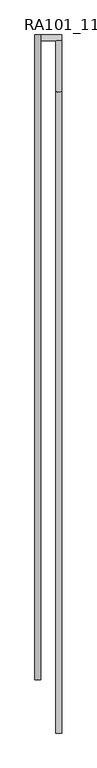
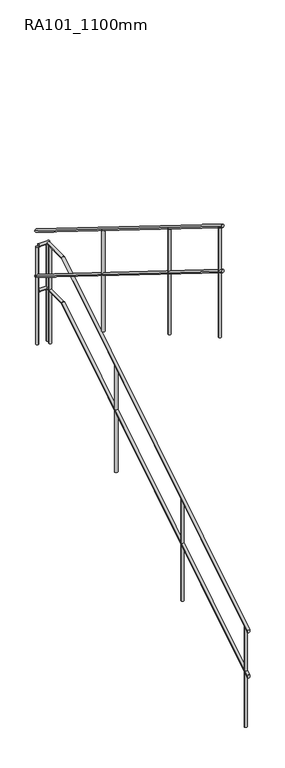
"""IFC4 building model written with IfcOpenShell, lengths in millimetres: railing geometry, RA101_1100mm."""

import ifcopenshell
import ifcopenshell.guid

model = None  # the IFC model being written
_history = None  # IfcOwnerHistory: only IFC2X3 demands one
_inside = {}  # id of a spatial element -> (the spatial element, [elements in it])
_under = {}  # id of a project, library or spatial element -> (it, [spatial elements below it])
_declared = {}  # id of a project -> (the project, [libraries it declares])
_typed = {}  # id of a type object -> (the type object, [elements of that type])
_made_of = {}  # id of a material, layer set ... -> (it, [elements and type objects made of it])


def new_model(schema):
    """Start an empty IFC model of exactly this schema.

    Asked for "IFC4X3", IfcOpenShell would pick the latest addendum, in which some entities
    have other attributes; the version numbers below select the first issue.
    IFC2X3 requires an IfcOwnerHistory on every rooted entity: one is made here for all.
    """
    global model, _history
    if schema == "IFC4X3":
        model = ifcopenshell.file(schema_version=(4, 3, 0, 0))
    else:
        model = ifcopenshell.file(schema=schema)
    _inside.clear()
    _under.clear()
    _declared.clear()
    _typed.clear()
    _made_of.clear()
    _history = None
    if model.schema == "IFC2X3":
        org = make("IfcOrganization", Name="unknown")
        user = make(
            "IfcPersonAndOrganization",
            ThePerson=make("IfcPerson", FamilyName="unknown"),
            TheOrganization=org,
        )
        app = make(
            "IfcApplication",
            ApplicationDeveloper=org,
            Version="unknown",
            ApplicationFullName="unknown",
            ApplicationIdentifier="unknown",
        )
        _history = make(
            "IfcOwnerHistory",
            OwningUser=user,
            OwningApplication=app,
            ChangeAction="ADDED",
            CreationDate=0,
        )
    return model


def make(cls, **values):
    """One entity of the class cls with the attributes given. An attribute that is None is left unset."""
    return model.create_entity(
        cls, **{name: value for name, value in values.items() if value is not None}
    )


def rooted(cls, **values):
    """An entity with a GlobalId (a new one), such as an element, a storey or a relation."""
    return make(cls, GlobalId=ifcopenshell.guid.new(), OwnerHistory=_history, **values)


def si_unit(unit_type, name, prefix=None):
    """IfcSIUnit, for example si_unit("LENGTHUNIT", "METRE", prefix="MILLI")."""
    return make("IfcSIUnit", UnitType=unit_type, Prefix=prefix, Name=name)


def assignment(units):
    """IfcUnitAssignment: the units of a project."""
    return None if units is None else make("IfcUnitAssignment", Units=units)


def point(xyz):
    """IfcCartesianPoint."""
    return None if xyz is None else make("IfcCartesianPoint", Coordinates=xyz)


def direction(xyz):
    """IfcDirection."""
    return None if xyz is None else make("IfcDirection", DirectionRatios=xyz)


def frame(location, z_axis=None, x_axis=None):
    """IfcAxis2Placement3D, a coordinate frame: its origin and axes. An axis left out is left unset."""
    return make(
        "IfcAxis2Placement3D",
        Location=point(location),
        Axis=direction(z_axis),
        RefDirection=direction(x_axis),
    )


def frame_2d(location, x_axis=None):
    """IfcAxis2Placement2D, a coordinate frame in the plane: its origin and x axis."""
    return make(
        "IfcAxis2Placement2D", Location=point(location), RefDirection=direction(x_axis)
    )


def origin():
    """The frame at (0, 0, 0) with its axes left unset."""
    return frame((0.0, 0.0, 0.0))


def place(relative_to, where):
    """IfcLocalPlacement: puts the frame where relative to a parent placement (None: the world)."""
    return make(
        "IfcLocalPlacement", PlacementRelTo=relative_to, RelativePlacement=where
    )


def context(
    kind, dimensions, precision=None, world=None, true_north=None, identifier=None
):
    """IfcGeometricRepresentationContext, for example the 3D "Model" context."""
    return make(
        "IfcGeometricRepresentationContext",
        ContextIdentifier=identifier,
        ContextType=kind,
        CoordinateSpaceDimension=dimensions,
        Precision=precision,
        WorldCoordinateSystem=world,
        TrueNorth=true_north,
    )


def project(units=None, contexts=None):
    """IfcProject with its units and contexts."""
    return rooted(
        "IfcProject",
        Name="project",
        RepresentationContexts=contexts,
        UnitsInContext=assignment(units),
    )


def spatial(cls, under=None, at=None, **own):
    """A site, building, storey or space (cls), placed at a placement, below another one or the project."""
    s = rooted(cls, ObjectPlacement=at, **own)
    if under is not None:
        _under.setdefault(under.id(), (under, []))[1].append(s)
    return s


def circle_curve(where, radius):
    """IfcCircle in the frame where."""
    return make("IfcCircle", Position=where, Radius=radius)


def ellipse_curve(where, semi_axis1, semi_axis2):
    """IfcEllipse in the frame where."""
    return make(
        "IfcEllipse", Position=where, SemiAxis1=semi_axis1, SemiAxis2=semi_axis2
    )


def trimmed(basis, trim1, trim2, sense, master):
    """IfcTrimmedCurve: the piece of a basis curve between two trims."""
    return make(
        "IfcTrimmedCurve",
        BasisCurve=basis,
        Trim1=trim1,
        Trim2=trim2,
        SenseAgreement=sense,
        MasterRepresentation=master,
    )


def segment(curve, same_sense, transition):
    """IfcCompositeCurveSegment."""
    return make(
        "IfcCompositeCurveSegment",
        Transition=transition,
        SameSense=same_sense,
        ParentCurve=curve,
    )


def composite_curve(segments, self_intersect=None):
    """IfcCompositeCurve: segments joined end to end."""
    return make("IfcCompositeCurve", Segments=segments, SelfIntersect=self_intersect)


def outline(outer, holes=None, kind="AREA"):
    """IfcArbitraryClosedProfileDef: a profile drawn as a closed curve; with holes, ...WithVoids."""
    if holes is None:
        return make("IfcArbitraryClosedProfileDef", ProfileType=kind, OuterCurve=outer)
    return make(
        "IfcArbitraryProfileDefWithVoids",
        ProfileType=kind,
        OuterCurve=outer,
        InnerCurves=holes,
    )


def extrude(swept, where, along, depth):
    """IfcExtrudedAreaSolid: the profile swept, set in the frame where, extruded along a direction by depth."""
    return make(
        "IfcExtrudedAreaSolid",
        SweptArea=swept,
        Position=where,
        ExtrudedDirection=direction(along),
        Depth=depth,
    )


def shape(context_of_items, identifier, shape_type, items):
    """IfcShapeRepresentation: the items that make up one representation, for example the "Body"."""
    return make(
        "IfcShapeRepresentation",
        ContextOfItems=context_of_items,
        RepresentationIdentifier=identifier,
        RepresentationType=shape_type,
        Items=items,
    )


def source(mapping_origin, context_of_items, identifier, shape_type, items):
    """IfcRepresentationMap: a shape defined once, which mapped items show again and again."""
    return make(
        "IfcRepresentationMap",
        MappingOrigin=mapping_origin,
        MappedRepresentation=shape(context_of_items, identifier, shape_type, items),
    )


def transform(
    local_origin,
    x_axis=None,
    y_axis=None,
    z_axis=None,
    scale=None,
    scale2=None,
    scale3=None,
    uniform=True,
):
    """IfcCartesianTransformationOperator3D, or its non-uniform kind. x_axis, y_axis, z_axis: its Axis1, 2, 3."""
    if uniform:
        return make(
            "IfcCartesianTransformationOperator3D",
            Axis1=direction(x_axis),
            Axis2=direction(y_axis),
            LocalOrigin=point(local_origin),
            Scale=scale,
            Axis3=direction(z_axis),
        )
    return make(
        "IfcCartesianTransformationOperator3DnonUniform",
        Axis1=direction(x_axis),
        Axis2=direction(y_axis),
        LocalOrigin=point(local_origin),
        Scale=scale,
        Axis3=direction(z_axis),
        Scale2=scale2,
        Scale3=scale3,
    )


def mapped(mapping_source, mapping_target):
    """IfcMappedItem: shows the shape of a source again, moved by a transform."""
    return make(
        "IfcMappedItem", MappingSource=mapping_source, MappingTarget=mapping_target
    )


def made_of(thing, what):
    """Note that an element or type object is made of a material, layer set ...; save() writes the relation."""
    if what is not None:
        _made_of.setdefault(what.id(), (what, []))[1].append(thing)
    return thing


def element(
    cls,
    number,
    at=None,
    inside=None,
    cuts=None,
    type_object=None,
    material=None,
    context=None,
    identifier="Body",
    shape_type=None,
    held_by="IfcProductDefinitionShape",
    body=None,
    shapes=None,
    **own,
):
    """One element of the class cls, such as IfcWall. Its Tag is "e" and its number.

    at: its placement. inside: the storey or other place that contains it. cuts: it is an
    opening in that element (IfcRelVoidsElement). A single representation is given by context,
    identifier, shape_type and body (its items); several are given by shapes. held_by: the class
    of the entity that holds the representations. save() writes the other relations.
    """
    e = rooted(cls, Tag="e%d" % number, ObjectPlacement=at, **own)
    if body is not None:
        shapes = [shape(context, identifier, shape_type, body)]
    if shapes is not None:
        e.Representation = make(held_by, Representations=shapes)
    if inside is not None:
        _inside.setdefault(inside.id(), (inside, []))[1].append(e)
    if cuts is not None:
        rooted(
            "IfcRelVoidsElement", RelatingBuildingElement=cuts, RelatedOpeningElement=e
        )
    if type_object is not None:
        _typed.setdefault(type_object.id(), (type_object, []))[1].append(e)
    return made_of(e, material)


def aggregate(whole, parts):
    """IfcRelAggregates: a whole, such as a stair, and the parts it consists of."""
    return rooted("IfcRelAggregates", RelatingObject=whole, RelatedObjects=parts)


def save(model, path):
    """Write the relations noted so far, then the file.

    IfcRelAggregates (storeys below a building ...), IfcRelContainedInSpatialStructure (elements
    in a storey), IfcRelDefinesByType, IfcRelAssociatesMaterial and IfcRelDeclares: one each for
    every whole, place, type object, material and project.
    """
    for whole, parts in _under.values():
        aggregate(whole, parts)
    for where, things in _inside.values():
        rooted(
            "IfcRelContainedInSpatialStructure",
            RelatedElements=things,
            RelatingStructure=where,
        )
    for kind, things in _typed.values():
        rooted("IfcRelDefinesByType", RelatedObjects=things, RelatingType=kind)
    for what, things in _made_of.values():
        rooted("IfcRelAssociatesMaterial", RelatedObjects=things, RelatingMaterial=what)
    for by, libraries in _declared.values():
        rooted("IfcRelDeclares", RelatingContext=by, RelatedDefinitions=libraries)
    model.write(path)


def plane_surface(at):
    """IfcPlane: the flat surface through the origin of the frame at, square to its z axis."""
    return make("IfcPlane", Position=at)


def cylinder_surface(at, radius):
    """IfcCylindricalSurface: all points at the distance radius from the z axis of the frame at."""
    return make("IfcCylindricalSurface", Position=at, Radius=radius)


def advanced_brep(points, edges, surfaces, faces):
    """IfcAdvancedBrep: a solid bounded by faces that lie on surfaces and meet in shared edges.

    An edge is (start, end): straight between two places in points (the first is 0);
    or (start, end, curve); or (start, end, curve, False) where it runs against its curve.
    A face is (place in surfaces, loops), or (place, loops, False) where it looks against
    its surface's normal. A loop lists edges by number (the first is 1), with a minus sign
    where the edge is run from its end to its start. The first loop is the outer one.
    """
    corners = [point(p) for p in points]
    vertices = [make("IfcVertexPoint", VertexGeometry=c) for c in corners]
    made = []
    for start, end, *more in edges:
        made.append(
            make(
                "IfcEdgeCurve",
                EdgeStart=vertices[start],
                EdgeEnd=vertices[end],
                EdgeGeometry=more[0] if more else make("IfcPolyline", Points=[corners[start], corners[end]]),
                SameSense=more[1] if len(more) > 1 else True,
            )
        )
    hull = []
    for where, loops, *sense in faces:
        bounds = []
        for j, loop in enumerate(loops):
            ring = [make("IfcOrientedEdge", EdgeElement=made[abs(k) - 1], Orientation=k > 0) for k in loop]
            bounds.append(
                make(
                    "IfcFaceOuterBound" if j == 0 else "IfcFaceBound",
                    Bound=make("IfcEdgeLoop", EdgeList=ring),
                    Orientation=True,
                )
            )
        hull.append(make("IfcAdvancedFace", Bounds=bounds, FaceSurface=surfaces[where], SameSense=sense[0] if sense else True))
    return make("IfcAdvancedBrep", Outer=make("IfcClosedShell", CfsFaces=hull))


def ra101_1100mm_1ac2519f(model_context):
    return source(origin(), model_context, "Body", "SolidModel", [
        advanced_brep(
        [(11545.1052251, 14699.5208589, 456.3396197), (11515.1052251, 14699.5208589, 456.3396197), (11545.1052251, 18329.5208589, 2547.0), (11515.1052251, 18329.5208589, 2547.0), (11545.1052251, 18063.8019306, 2547.0), (11515.1052251, 18063.8019306, 2547.0)],
        [
            (0, 1, ellipse_curve(frame((11530.1052251, 14699.5208589, 456.3396197), z_axis=(0.0, -1.0, 0.0), x_axis=(0.0, 0.0, -1.0)), 17.6603803, 15.0)),
            (1, 0, ellipse_curve(frame((11530.1052251, 14699.5208589, 456.3396197), z_axis=(0.0, -1.0, 0.0), x_axis=(0.0, 0.0, -1.0)), 17.6603803, 15.0)),
            (2, 3, circle_curve(frame((11530.1052251, 18329.5208589, 2547.0), z_axis=(0.0, 1.0, 0.0), x_axis=(-1.0, 0.0, 0.0)), 15.0)),
            (3, 2, circle_curve(frame((11530.1052251, 18329.5208589, 2547.0), z_axis=(0.0, 1.0, 0.0), x_axis=(-1.0, 0.0, 0.0)), 15.0)),
            (0, 4),
            (4, 5, ellipse_curve(frame((11530.1052251, 18063.8019306, 2547.0), z_axis=(0.0, -0.9616025257983003, -0.2744459552959912), x_axis=(0.0, 0.2744459552959914, -0.9616025257983002)), 15.5989607, 15.0)),
            (5, 1),
            (5, 4, ellipse_curve(frame((11530.1052251, 18063.8019306, 2547.0), z_axis=(0.0, -0.9616025257983003, -0.2744459552959912), x_axis=(0.0, 0.2744459552959914, -0.9616025257983002)), 15.5989607, 15.0)),
            (4, 2),
            (3, 5),
        ],
        [
            plane_surface(frame((11530.1052251, 14699.5208589, 474.0), z_axis=(0.0, -1.0, 0.0), x_axis=(0.0, 0.0, 1.0))),
            plane_surface(frame((11530.1052251, 18329.5208589, 2562.0), z_axis=(0.0, 1.0, 0.0), x_axis=(0.0, 0.0, 1.0))),
            cylinder_surface(frame((11530.1052251, 14707.4380966, 461.2596175), z_axis=(0.0, -0.8493588352433417, -0.5278158476155052), x_axis=(-1.0, 0.0, 0.0)), 15.0),
            cylinder_surface(frame((11530.1052251, 18059.5208589, 2547.0), z_axis=(0.0, -1.0, 0.0), x_axis=(-1.0, 0.0, 0.0)), 15.0),
        ],
        [
            (0, [[1, 2]]),
            (1, [[3, 4]]),
            (2, [[-1, 5, 6, 7]]),
            (2, [[-2, -7, 8, -5]]),
            (3, [[-6, 9, -4, 10]]),
            (3, [[-8, -10, -3, -9]]),
        ],
    ),
        advanced_brep(
        [(11545.1052251, 18359.5208589, 2547.0), (11545.1052251, 18329.5208589, 2547.0), (11435.1052251, 18359.5208589, 2547.0), (11435.1052251, 18329.5208589, 2547.0)],
        [
            (0, 1, circle_curve(frame((11545.1052251, 18344.5208589, 2547.0), z_axis=(1.0, 0.0, 0.0), x_axis=(0.0, -1.0, 0.0)), 15.0)),
            (1, 0, circle_curve(frame((11545.1052251, 18344.5208589, 2547.0), z_axis=(1.0, 0.0, 0.0), x_axis=(0.0, -1.0, 0.0)), 15.0)),
            (2, 3, circle_curve(frame((11435.1052251, 18344.5208589, 2547.0), z_axis=(-1.0, 0.0, 0.0), x_axis=(0.0, -1.0, 0.0)), 15.0)),
            (3, 2, circle_curve(frame((11435.1052251, 18344.5208589, 2547.0), z_axis=(-1.0, 0.0, 0.0), x_axis=(0.0, -1.0, 0.0)), 15.0)),
            (0, 2),
            (3, 1),
        ],
        [
            plane_surface(frame((11545.1052251, 18344.5208589, 2562.0), z_axis=(1.0, 0.0, 0.0), x_axis=(0.0, -1.0, 0.0))),
            plane_surface(frame((11435.1052251, 18344.5208589, 2562.0), z_axis=(-1.0, 0.0, 0.0), x_axis=(0.0, -1.0, 0.0))),
            cylinder_surface(frame((11545.1052251, 18344.5208589, 2547.0), z_axis=(1.0, 0.0, 0.0), x_axis=(0.0, -1.0, 0.0)), 15.0),
        ],
        [
            (0, [[1, 2]]),
            (1, [[3, 4]]),
            (2, [[-1, 5, -4, 6]]),
            (2, [[-2, -6, -3, -5]]),
        ],
    ),
        advanced_brep(
        [(11405.1052251, 18359.5208589, 2705.9110483), (11435.1052251, 18359.5208589, 2705.9110483), (11405.1052251, 14979.5208589, 4806.3396197), (11435.1052251, 14979.5208589, 4806.3396197)],
        [
            (0, 1, ellipse_curve(frame((11420.1052251, 18359.5208589, 2705.9110483), z_axis=(0.0, 1.0, 0.0), x_axis=(0.0, 0.0, -1.0)), 17.6603803, 15.0)),
            (1, 0, ellipse_curve(frame((11420.1052251, 18359.5208589, 2705.9110483), z_axis=(0.0, 1.0, 0.0), x_axis=(0.0, 0.0, -1.0)), 17.6603803, 15.0)),
            (2, 3, ellipse_curve(frame((11420.1052251, 14979.5208589, 4806.3396197), z_axis=(0.0, -1.0, 0.0), x_axis=(0.0, 0.0, -1.0)), 17.6603803, 15.0)),
            (3, 2, ellipse_curve(frame((11420.1052251, 14979.5208589, 4806.3396197), z_axis=(0.0, -1.0, 0.0), x_axis=(0.0, 0.0, -1.0)), 17.6603803, 15.0)),
            (0, 2),
            (3, 1),
        ],
        [
            plane_surface(frame((11420.1052251, 18359.5208589, 2723.5714286), z_axis=(0.0, 1.0, 0.0), x_axis=(0.0, 0.0, -1.0))),
            plane_surface(frame((11420.1052251, 14979.5208589, 4824.0), z_axis=(0.0, -1.0, 0.0), x_axis=(0.0, 0.0, -1.0))),
            cylinder_surface(frame((11420.1052251, 18351.6036212, 2710.831046), z_axis=(0.0, 0.8493588352433417, -0.5278158476155052), x_axis=(1.0, 0.0, 0.0)), 15.0),
        ],
        [
            (0, [[1, 2]]),
            (1, [[3, 4]]),
            (2, [[-1, 5, -4, 6]]),
            (2, [[-2, -6, -3, -5]]),
        ],
    ),
        advanced_brep(
        [(11545.1052251, 14699.5208589, 956.3396197), (11515.1052251, 14699.5208589, 956.3396197), (11545.1052251, 18063.8019306, 3047.0), (11515.1052251, 18063.8019306, 3047.0), (11545.1052251, 18329.5208589, 3047.0), (11515.1052251, 18329.5208589, 3047.0)],
        [
            (0, 1, ellipse_curve(frame((11530.1052251, 14699.5208589, 956.3396197), z_axis=(0.0, -1.0, 0.0), x_axis=(0.0, 0.0, -1.0)), 17.6603803, 15.0)),
            (1, 0, ellipse_curve(frame((11530.1052251, 14699.5208589, 956.3396197), z_axis=(0.0, -1.0, 0.0), x_axis=(0.0, 0.0, -1.0)), 17.6603803, 15.0)),
            (0, 2),
            (2, 3, ellipse_curve(frame((11530.1052251, 18063.8019306, 3047.0), z_axis=(0.0, -0.9616025257983003, -0.2744459552959912), x_axis=(0.0, 0.2744459552959914, -0.9616025257983002)), 15.5989607, 15.0)),
            (3, 1),
            (3, 2, ellipse_curve(frame((11530.1052251, 18063.8019306, 3047.0), z_axis=(0.0, -0.9616025257983003, -0.2744459552959912), x_axis=(0.0, 0.2744459552959914, -0.9616025257983002)), 15.5989607, 15.0)),
            (4, 5, circle_curve(frame((11530.1052251, 18329.5208589, 3047.0), z_axis=(0.0, 1.0, 0.0), x_axis=(-1.0, 0.0, 0.0)), 15.0)),
            (5, 4, circle_curve(frame((11530.1052251, 18329.5208589, 3047.0), z_axis=(0.0, 1.0, 0.0), x_axis=(-1.0, 0.0, 0.0)), 15.0)),
            (2, 4),
            (5, 3),
        ],
        [
            plane_surface(frame((11530.1052251, 14699.5208589, 974.0), z_axis=(0.0, -1.0, 0.0), x_axis=(0.0, 0.0, 1.0))),
            cylinder_surface(frame((11530.1052251, 14707.4380966, 961.2596175), z_axis=(0.0, -0.8493588352433417, -0.5278158476155052), x_axis=(-1.0, 0.0, 0.0)), 15.0),
            plane_surface(frame((11530.1052251, 18329.5208589, 3062.0), z_axis=(0.0, 1.0, 0.0), x_axis=(0.0, 0.0, 1.0))),
            cylinder_surface(frame((11530.1052251, 18059.5208589, 3047.0), z_axis=(0.0, -1.0, 0.0), x_axis=(-1.0, 0.0, 0.0)), 15.0),
        ],
        [
            (0, [[1, 2]]),
            (1, [[-1, 3, 4, 5]]),
            (1, [[-2, -5, 6, -3]]),
            (2, [[7, 8]]),
            (3, [[-4, 9, -8, 10]]),
            (3, [[-6, -10, -7, -9]]),
        ],
    ),
        advanced_brep(
        [(11545.1052251, 18359.5208589, 3047.0), (11545.1052251, 18329.5208589, 3047.0), (11435.1052251, 18359.5208589, 3047.0), (11435.1052251, 18329.5208589, 3047.0)],
        [
            (0, 1, circle_curve(frame((11545.1052251, 18344.5208589, 3047.0), z_axis=(1.0, 0.0, 0.0), x_axis=(0.0, -1.0, 0.0)), 15.0)),
            (1, 0, circle_curve(frame((11545.1052251, 18344.5208589, 3047.0), z_axis=(1.0, 0.0, 0.0), x_axis=(0.0, -1.0, 0.0)), 15.0)),
            (2, 3, circle_curve(frame((11435.1052251, 18344.5208589, 3047.0), z_axis=(-1.0, 0.0, 0.0), x_axis=(0.0, -1.0, 0.0)), 15.0)),
            (3, 2, circle_curve(frame((11435.1052251, 18344.5208589, 3047.0), z_axis=(-1.0, 0.0, 0.0), x_axis=(0.0, -1.0, 0.0)), 15.0)),
            (0, 2),
            (3, 1),
        ],
        [
            plane_surface(frame((11545.1052251, 18344.5208589, 3062.0), z_axis=(1.0, 0.0, 0.0), x_axis=(0.0, -1.0, 0.0))),
            plane_surface(frame((11435.1052251, 18344.5208589, 3062.0), z_axis=(-1.0, 0.0, 0.0), x_axis=(0.0, -1.0, 0.0))),
            cylinder_surface(frame((11545.1052251, 18344.5208589, 3047.0), z_axis=(1.0, 0.0, 0.0), x_axis=(0.0, -1.0, 0.0)), 15.0),
        ],
        [
            (0, [[1, 2]]),
            (1, [[3, 4]]),
            (2, [[-1, 5, -4, 6]]),
            (2, [[-2, -6, -3, -5]]),
        ],
    ),
        advanced_brep(
        [(11405.1052251, 18359.5208589, 3205.9110483), (11435.1052251, 18359.5208589, 3205.9110483), (11405.1052251, 14979.5208589, 5306.3396197), (11435.1052251, 14979.5208589, 5306.3396197)],
        [
            (0, 1, ellipse_curve(frame((11420.1052251, 18359.5208589, 3205.9110483), z_axis=(0.0, 1.0, 0.0), x_axis=(0.0, 0.0, -1.0)), 17.6603803, 15.0)),
            (1, 0, ellipse_curve(frame((11420.1052251, 18359.5208589, 3205.9110483), z_axis=(0.0, 1.0, 0.0), x_axis=(0.0, 0.0, -1.0)), 17.6603803, 15.0)),
            (2, 3, ellipse_curve(frame((11420.1052251, 14979.5208589, 5306.3396197), z_axis=(0.0, -1.0, 0.0), x_axis=(0.0, 0.0, -1.0)), 17.6603803, 15.0)),
            (3, 2, ellipse_curve(frame((11420.1052251, 14979.5208589, 5306.3396197), z_axis=(0.0, -1.0, 0.0), x_axis=(0.0, 0.0, -1.0)), 17.6603803, 15.0)),
            (0, 2),
            (3, 1),
        ],
        [
            plane_surface(frame((11420.1052251, 18359.5208589, 3223.5714286), z_axis=(0.0, 1.0, 0.0), x_axis=(0.0, 0.0, -1.0))),
            plane_surface(frame((11420.1052251, 14979.5208589, 5324.0), z_axis=(0.0, -1.0, 0.0), x_axis=(0.0, 0.0, -1.0))),
            cylinder_surface(frame((11420.1052251, 18351.6036212, 3210.831046), z_axis=(0.0, 0.8493588352433417, -0.5278158476155052), x_axis=(1.0, 0.0, 0.0)), 15.0),
        ],
        [
            (0, [[1, 2]]),
            (1, [[3, 4]]),
            (2, [[-1, 5, -4, 6]]),
            (2, [[-2, -6, -3, -5]]),
        ],
    ),
        extrude(outline(composite_curve([segment(trimmed(circle_curve(frame_2d((11420.1052251, 15944.5208589)), 15.0), [point((11435.1052251, 15944.5208589))], [point((11405.1052251, 15944.5208589))], False, "CARTESIAN"), True, "CONTINUOUS"), segment(trimmed(circle_curve(frame_2d((11420.1052251, 15944.5208589)), 15.0), [point((11405.1052251, 15944.5208589))], [point((11435.1052251, 15944.5208589))], False, "CARTESIAN"), True, "CONTINUOUS")], self_intersect=False)), frame((0.0, 0.0, 3528.0), z_axis=(0.0, 0.0, 1.0), x_axis=(1.0, 0.0, 0.0)), (0.0, 0.0, 1.0), 1166.3214286),
        extrude(outline(composite_curve([segment(trimmed(circle_curve(frame_2d((11420.1052251, 17144.5208589)), 15.0), [point((11435.1052251, 17144.5208589))], [point((11405.1052251, 17144.5208589))], False, "CARTESIAN"), True, "CONTINUOUS"), segment(trimmed(circle_curve(frame_2d((11420.1052251, 17144.5208589)), 15.0), [point((11405.1052251, 17144.5208589))], [point((11435.1052251, 17144.5208589))], False, "CARTESIAN"), True, "CONTINUOUS")], self_intersect=False)), frame((0.0, 0.0, 2832.0), z_axis=(0.0, 0.0, 1.0), x_axis=(1.0, 0.0, 0.0)), (0.0, 0.0, 1.0), 1116.6071429),
        extrude(outline(composite_curve([segment(trimmed(circle_curve(frame_2d((11530.1052251, 18299.5208589)), 15.0), [point((11515.1052251, 18299.5208589))], [point((11545.1052251, 18299.5208589))], False, "CARTESIAN"), True, "CONTINUOUS"), segment(trimmed(circle_curve(frame_2d((11530.1052251, 18299.5208589)), 15.0), [point((11545.1052251, 18299.5208589))], [point((11515.1052251, 18299.5208589))], False, "CARTESIAN"), True, "CONTINUOUS")], self_intersect=False)), frame((0.0, 0.0, 1962.0), z_axis=(0.0, 0.0, 1.0), x_axis=(1.0, 0.0, 0.0)), (0.0, 0.0, 1.0), 1070.0),
        extrude(outline(composite_curve([segment(trimmed(circle_curve(frame_2d((11530.1052251, 17099.5208589)), 15.0), [point((11515.1052251, 17099.5208589))], [point((11545.1052251, 17099.5208589))], False, "CARTESIAN"), True, "CONTINUOUS"), segment(trimmed(circle_curve(frame_2d((11530.1052251, 17099.5208589)), 15.0), [point((11545.1052251, 17099.5208589))], [point((11515.1052251, 17099.5208589))], False, "CARTESIAN"), True, "CONTINUOUS")], self_intersect=False)), frame((0.0, 0.0, 1266.0), z_axis=(0.0, 0.0, 1.0), x_axis=(1.0, 0.0, 0.0)), (0.0, 0.0, 1.0), 1169.4285714),
        extrude(outline(composite_curve([segment(trimmed(circle_curve(frame_2d((11530.1052251, 15899.5208589)), 15.0), [point((11515.1052251, 15899.5208589))], [point((11545.1052251, 15899.5208589))], False, "CARTESIAN"), True, "CONTINUOUS"), segment(trimmed(circle_curve(frame_2d((11530.1052251, 15899.5208589)), 15.0), [point((11545.1052251, 15899.5208589))], [point((11515.1052251, 15899.5208589))], False, "CARTESIAN"), True, "CONTINUOUS")], self_intersect=False)), frame((0.0, 0.0, 570.0), z_axis=(0.0, 0.0, 1.0), x_axis=(1.0, 0.0, 0.0)), (0.0, 0.0, 1.0), 1119.7142857),
        extrude(outline(composite_curve([segment(trimmed(circle_curve(frame_2d((11420.1052251, 18344.5208589)), 15.0), [point((11420.1052251, 18329.5208589))], [point((11420.1052251, 18359.5208589))], False, "CARTESIAN"), True, "CONTINUOUS"), segment(trimmed(circle_curve(frame_2d((11420.1052251, 18344.5208589)), 15.0), [point((11420.1052251, 18359.5208589))], [point((11420.1052251, 18329.5208589))], False, "CARTESIAN"), True, "CONTINUOUS")], self_intersect=False)), frame((0.0, 0.0, 1962.0), z_axis=(0.0, 0.0, 1.0), x_axis=(1.0, 0.0, 0.0)), (0.0, 0.0, 1.0), 1070.0),
        extrude(outline(composite_curve([segment(trimmed(circle_curve(frame_2d((11530.1052251, 18344.5208589)), 15.0), [point((11515.1052251, 18344.5208589))], [point((11545.1052251, 18344.5208589))], False, "CARTESIAN"), True, "CONTINUOUS"), segment(trimmed(circle_curve(frame_2d((11530.1052251, 18344.5208589)), 15.0), [point((11545.1052251, 18344.5208589))], [point((11515.1052251, 18344.5208589))], False, "CARTESIAN"), True, "CONTINUOUS")], self_intersect=False)), frame((0.0, 0.0, 1962.0), z_axis=(0.0, 0.0, 1.0), x_axis=(1.0, 0.0, 0.0)), (0.0, 0.0, 1.0), 1070.0),
        extrude(outline(composite_curve([segment(trimmed(circle_curve(frame_2d((11420.1052251, 15029.5208589)), 15.0), [point((11435.1052251, 15029.5208589))], [point((11405.1052251, 15029.5208589))], False, "CARTESIAN"), True, "CONTINUOUS"), segment(trimmed(circle_curve(frame_2d((11420.1052251, 15029.5208589)), 15.0), [point((11405.1052251, 15029.5208589))], [point((11435.1052251, 15029.5208589))], False, "CARTESIAN"), True, "CONTINUOUS")], self_intersect=False)), frame((0.0, 0.0, 4050.0), z_axis=(0.0, 0.0, 1.0), x_axis=(1.0, 0.0, 0.0)), (0.0, 0.0, 1.0), 1212.9285714),
        extrude(outline(composite_curve([segment(trimmed(circle_curve(frame_2d((11530.1052251, 14749.5208589)), 15.0), [point((11515.1052251, 14749.5208589))], [point((11545.1052251, 14749.5208589))], False, "CARTESIAN"), True, "CONTINUOUS"), segment(trimmed(circle_curve(frame_2d((11530.1052251, 14749.5208589)), 15.0), [point((11545.1052251, 14749.5208589))], [point((11515.1052251, 14749.5208589))], False, "CARTESIAN"), True, "CONTINUOUS")], self_intersect=False)), frame((0.0, 0.0, -126.0), z_axis=(0.0, 0.0, 1.0), x_axis=(1.0, 0.0, 0.0)), (0.0, 0.0, 1.0), 1101.0714286),
    ])


if __name__ == "__main__":
    model = new_model("IFC4")
    model_context = context("Model", 3, world=origin())
    ifc_project = project(units=[si_unit("LENGTHUNIT", "METRE", prefix="MILLI")], contexts=[model_context])
    site = spatial("IfcSite", under=ifc_project)
    building = spatial("IfcBuilding", under=site)
    placement = place(None, origin())
    ra101_1100mm_shape = ra101_1100mm_1ac2519f(model_context)
    element("IfcRailing", 1, ObjectType="RA101_1100mm", at=placement, inside=building, context=model_context, shape_type="MappedRepresentation", body=[
        mapped(ra101_1100mm_shape, transform((0.0, 0.0, 0.0), x_axis=(1.0, 0.0, 0.0), y_axis=(0.0, 1.0, 0.0), z_axis=(0.0, 0.0, 1.0))),
    ])
    save(model, "model.ifc")

# Revit data of these elements
# Project information
#   Building Name = "MAIN GATE SECURITY BUILDING"
#   Project Status = "Project Status"
#   Client Name = "현대엔지니어링"
#   Project Address = "서울시 종로구 율곡로 75(계동)"
#   Project Name = "Therma Visayas Energy Project"
#   Project Number = "-"
